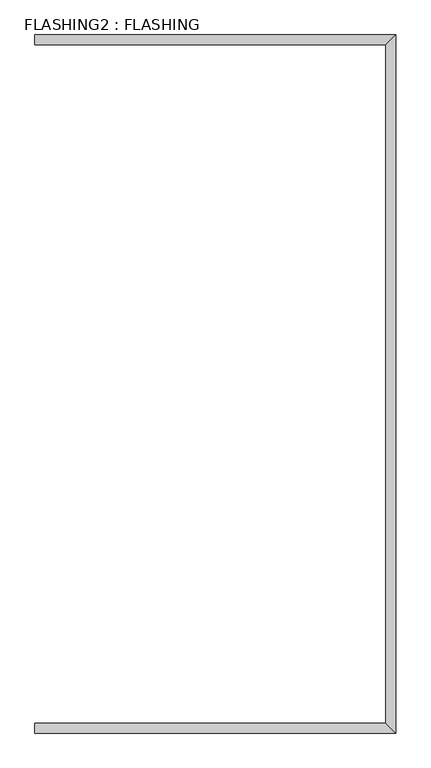
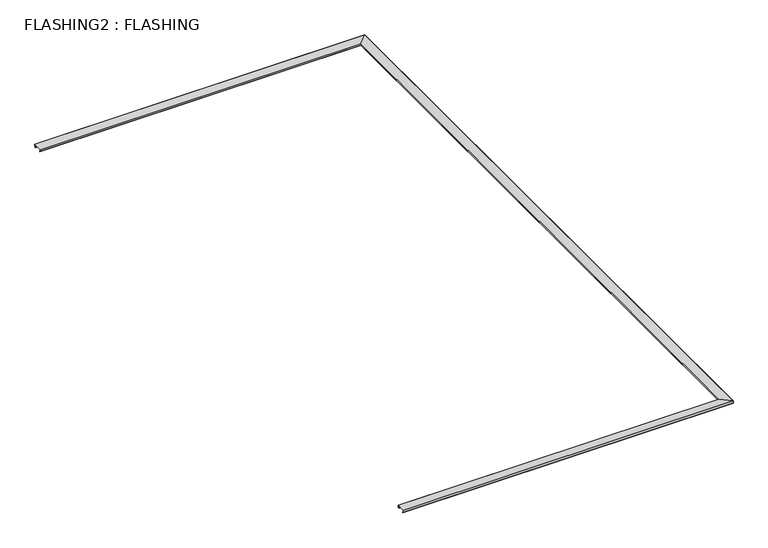
"""IFC4 building model written with IfcOpenShell, lengths in millimetres: proxy geometry, FLASHING2 : FLASHING."""

from ifc_helpers import new_model, si_unit, origin, place, context, project, spatial, faceted_brep, source, transform, mapped, element, save


def flashing2_flashing_8f2ab91a(model_context):
    return source(origin(), model_context, "Body", "Brep", [
        faceted_brep([(50865.0, 39914.5208589, 7739.9720055), (50865.0, 39914.5208589, 7724.9720055), (50865.0, 20084.5208589, 7724.9720055), (50865.0, 20084.5208589, 7739.9720055), (50866.0, 39915.5208589, 7750.9720055), (50866.0, 39915.5208589, 7739.9720055), (50866.0, 20083.5208589, 7739.9720055), (50866.0, 20083.5208589, 7750.9720055), (50894.0, 39943.5208589, 7819.1280996), (50894.0, 39943.5208589, 7750.9720055), (50894.0, 20055.5208589, 7750.9720055), (50894.0, 20055.5208589, 7819.1280996), (50611.0, 39660.5208589, 7808.0300604), (50611.0, 20338.5208589, 7808.0300604), (50611.0, 39660.5208589, 7750.9720055), (50611.0, 20338.5208589, 7750.9720055), (50639.0, 39688.5208589, 7739.9720055), (50639.0, 39688.5208589, 7750.9720055), (50639.0, 20310.5208589, 7750.9720055), (50639.0, 20310.5208589, 7739.9720055), (50640.0, 39689.5208589, 7724.9720055), (50640.0, 39689.5208589, 7739.9720055), (50640.0, 20309.5208589, 7739.9720055), (50640.0, 20309.5208589, 7724.9720055), (50638.0, 39687.5208589, 7749.9720055), (50638.0, 39687.5208589, 7724.9720055), (50638.0, 20311.5208589, 7724.9720055), (50638.0, 20311.5208589, 7749.9720055), (50610.0, 39659.5208589, 7808.9916134), (50610.0, 39659.5208589, 7749.9720055), (50610.0, 20339.5208589, 7749.9720055), (50610.0, 20339.5208589, 7808.9916134), (50895.0, 39944.5208589, 7820.168084), (50895.0, 20054.5208589, 7820.168084), (50895.0, 39944.5208589, 7749.9720055), (50895.0, 20054.5208589, 7749.9720055), (50867.0, 39916.5208589, 7724.9720055), (50867.0, 39916.5208589, 7749.9720055), (50867.0, 20082.5208589, 7749.9720055), (50867.0, 20082.5208589, 7724.9720055), (40619.0, 20084.5208589, 7724.9720055), (40619.0, 20084.5208589, 7739.9720055), (40619.0, 20083.5208589, 7739.9720055), (40619.0, 20083.5208589, 7750.9720055), (40619.0, 20055.5208589, 7750.9720055), (40619.0, 20055.5208589, 7819.1280996), (40619.0, 20338.5208589, 7808.0300604), (40619.0, 20338.5208589, 7750.9720055), (40619.0, 20310.5208589, 7750.9720055), (40619.0, 20310.5208589, 7739.9720055), (40619.0, 20309.5208589, 7739.9720055), (40619.0, 20309.5208589, 7724.9720055), (40619.0, 20311.5208589, 7724.9720055), (40619.0, 20311.5208589, 7749.9720055), (40619.0, 20339.5208589, 7749.9720055), (40619.0, 20339.5208589, 7808.9916134), (40619.0, 20054.5208589, 7820.168084), (40619.0, 20054.5208589, 7749.9720055), (40619.0, 20082.5208589, 7749.9720055), (40619.0, 20082.5208589, 7724.9720055), (40619.0, 39914.5208589, 7739.9720055), (40619.0, 39914.5208589, 7724.9720055), (40619.0, 39915.5208589, 7739.9720055), (40619.0, 39915.5208589, 7750.9720055), (40619.0, 39943.5208589, 7750.9720055), (40619.0, 39943.5208589, 7819.1280996), (40619.0, 39660.5208589, 7808.0300604), (40619.0, 39660.5208589, 7750.9720055), (40619.0, 39688.5208589, 7750.9720055), (40619.0, 39688.5208589, 7739.9720055), (40619.0, 39689.5208589, 7739.9720055), (40619.0, 39689.5208589, 7724.9720055), (40619.0, 39687.5208589, 7724.9720055), (40619.0, 39687.5208589, 7749.9720055), (40619.0, 39659.5208589, 7749.9720055), (40619.0, 39659.5208589, 7808.9916134), (40619.0, 39944.5208589, 7820.168084), (40619.0, 39944.5208589, 7749.9720055), (40619.0, 39916.5208589, 7749.9720055), (40619.0, 39916.5208589, 7724.9720055)], [[[0, 1, 2, 3]], [[4, 5, 6, 7]], [[8, 9, 10, 11]], [[12, 8, 11, 13]], [[14, 12, 13, 15]], [[16, 17, 18, 19]], [[20, 21, 22, 23]], [[24, 25, 26, 27]], [[28, 29, 30, 31]], [[32, 28, 31, 33]], [[34, 32, 33, 35]], [[36, 37, 38, 39]], [[3, 2, 40, 41]], [[7, 6, 42, 43]], [[11, 10, 44, 45]], [[13, 11, 45, 46]], [[15, 13, 46, 47]], [[19, 18, 48, 49]], [[23, 22, 50, 51]], [[27, 26, 52, 53]], [[31, 30, 54, 55]], [[33, 31, 55, 56]], [[35, 33, 56, 57]], [[39, 38, 58, 59]], [[60, 61, 1, 0]], [[62, 60, 0, 3, 41, 42, 6, 5]], [[63, 62, 5, 4]], [[64, 63, 4, 7, 43, 44, 10, 9]], [[65, 64, 9, 8]], [[66, 65, 8, 12]], [[67, 66, 12, 14]], [[68, 67, 14, 15, 47, 48, 18, 17]], [[69, 68, 17, 16]], [[70, 69, 16, 19, 49, 50, 22, 21]], [[71, 70, 21, 20]], [[72, 71, 20, 23, 51, 52, 26, 25]], [[73, 72, 25, 24]], [[74, 73, 24, 27, 53, 54, 30, 29]], [[75, 74, 29, 28]], [[76, 75, 28, 32]], [[77, 76, 32, 34]], [[78, 77, 34, 35, 57, 58, 38, 37]], [[79, 78, 37, 36]], [[61, 79, 36, 39, 59, 40, 2, 1]], [[61, 60, 62, 63, 64, 65, 66, 67, 68, 69, 70, 71, 72, 73, 74, 75, 76, 77, 78, 79]], [[40, 59, 58, 57, 56, 55, 54, 53, 52, 51, 50, 49, 48, 47, 46, 45, 44, 43, 42, 41]]]),
    ])


if __name__ == "__main__":
    model = new_model("IFC4")
    model_context = context("Model", 3, world=origin())
    ifc_project = project(units=[si_unit("LENGTHUNIT", "METRE", prefix="MILLI")], contexts=[model_context])
    site = spatial("IfcSite", under=ifc_project)
    building = spatial("IfcBuilding", under=site)
    placement = place(None, origin())
    flashing2_flashing_shape = flashing2_flashing_8f2ab91a(model_context)
    element("IfcBuildingElementProxy", 1, Name="FLASHING2 : FLASHING", ObjectType="FLASHING2 : FLASHING", at=placement, inside=building, context=model_context, shape_type="MappedRepresentation", body=[
        mapped(flashing2_flashing_shape, transform((0.0, 0.0, 0.0), x_axis=(1.0, 0.0, 0.0), y_axis=(0.0, 1.0, 0.0), z_axis=(0.0, 0.0, 1.0))),
    ])
    save(model, "model.ifc")
